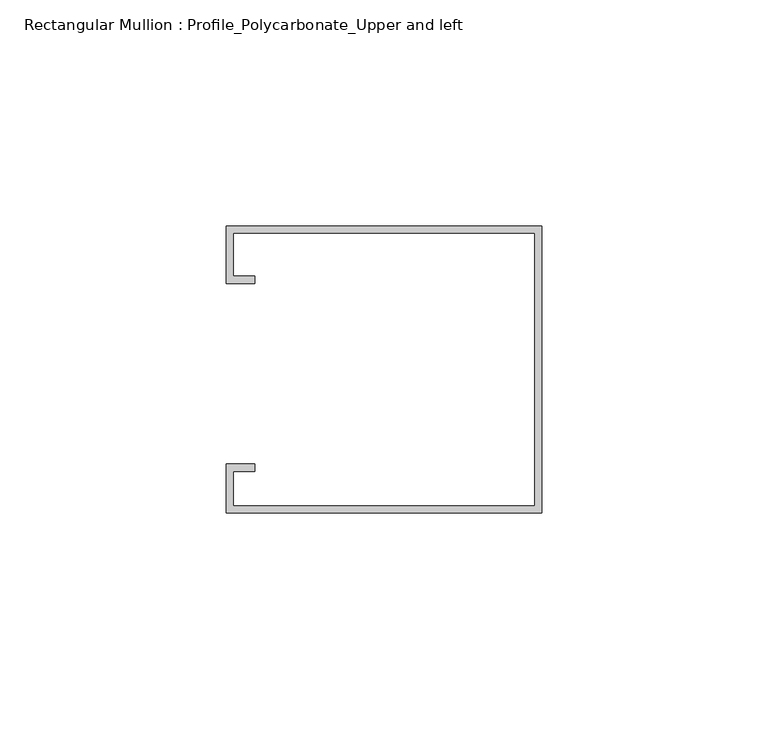
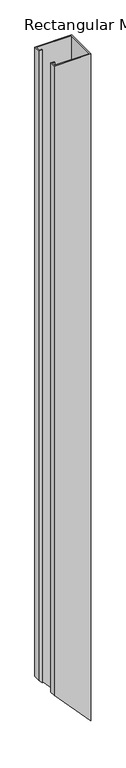
"""IFC4 building model written with IfcOpenShell, lengths in millimetres: member geometry, Rectangular Mullion : Profile_Polycarbonate_Upper and left."""

from ifc_helpers import new_model, si_unit, origin, place, context, project, spatial, faceted_brep, source, transform, mapped, element, save


def rectangular_mullion_profile_polycarbonate_upper_and_left_c3c58ff7(model_context):
    return source(origin(), model_context, "Body", "Brep", [
        faceted_brep([(0.0, 32.7, 0.0), (-69.85, 32.7, 0.0), (-69.85, 20.0, 0.0), (-63.5, 20.0, 0.0), (-63.5, 21.5875, 0.0), (-68.2625, 21.5875, 0.0), (-68.2625, 31.1125, 0.0), (-1.5875, 31.1125, 0.0), (-1.5875, -29.2125, 0.0), (-68.2625, -29.2125, 0.0), (-68.2625, -21.5875, 0.0), (-63.5, -21.5875, 0.0), (-63.5, -20.0, 0.0), (-69.85, -20.0, 0.0), (-69.85, -30.8, 0.0), (0.0, -30.8, 0.0), (0.0, 32.7, -1345.3170334), (-69.85, 32.7, -1269.404085), (-69.85, 20.0, -1269.404085), (-63.5, 20.0, -1276.3052621), (-63.5, 21.5875, -1276.3052621), (-68.2625, 21.5875, -1271.1293793), (-68.2625, 31.1125, -1271.1293793), (-1.5875, 31.1125, -1343.5917391), (-1.5875, -29.2125, -1343.5917391), (-68.2625, -29.2125, -1271.1293793), (-68.2625, -21.5875, -1271.1293793), (-63.5, -21.5875, -1276.3052621), (-63.5, -20.0, -1276.3052621), (-69.85, -20.0, -1269.404085), (-69.85, -30.8, -1269.404085), (0.0, -30.8, -1345.3170334)], [[[0, 1, 2, 3, 4, 5, 6, 7, 8, 9, 10, 11, 12, 13, 14, 15]], [[1, 0, 16, 17]], [[2, 1, 17, 18]], [[3, 2, 18, 19]], [[4, 3, 19, 20]], [[5, 4, 20, 21]], [[6, 5, 21, 22]], [[7, 6, 22, 23]], [[8, 7, 23, 24]], [[9, 8, 24, 25]], [[10, 9, 25, 26]], [[11, 10, 26, 27]], [[12, 11, 27, 28]], [[13, 12, 28, 29]], [[14, 13, 29, 30]], [[15, 14, 30, 31]], [[0, 15, 31, 16]], [[16, 31, 30, 29, 28, 27, 26, 25, 24, 23, 22, 21, 20, 19, 18, 17]]]),
    ])


if __name__ == "__main__":
    model = new_model("IFC4")
    model_context = context("Model", 3, world=origin())
    ifc_project = project(units=[si_unit("LENGTHUNIT", "METRE", prefix="MILLI")], contexts=[model_context])
    site = spatial("IfcSite", under=ifc_project)
    building = spatial("IfcBuilding", under=site)
    placement = place(None, origin())
    rectangular_mullion_profile_polycarbonate_upper_and_left_shape = rectangular_mullion_profile_polycarbonate_upper_and_left_c3c58ff7(model_context)
    element("IfcMember", 1, ObjectType="Rectangular Mullion : Profile_Polycarbonate_Upper and left", at=placement, inside=building, context=model_context, shape_type="MappedRepresentation", body=[
        mapped(rectangular_mullion_profile_polycarbonate_upper_and_left_shape, transform((0.0, 0.0, 0.0), x_axis=(1.0, 0.0, 0.0), y_axis=(0.0, 1.0, 0.0), z_axis=(0.0, 0.0, 1.0))),
    ])
    save(model, "model.ifc")

# Revit data of these elements
# Type "Rectangular Mullion : Profile_Polycarbonate_Upper and left"
#   built-in parameter 1007322 = 0.208333 (stored number, unit not read)
#   built-in parameter 1007321 = 0.00520833 (stored number, unit not read)
#   built-in parameter 1007320 = 0 (stored number, unit not read)
# Element 1 (IfcMember, "Rectangular Mullion : Profile_Polycarbonate_Upper and left")
#   Materials on its faces: "ALUMINUM PROFILE AT POLYCARBONATE PANEL"
# Materials
#   "ALUMINUM PROFILE AT POLYCARBONATE PANEL": class "Metal", colour RGB 244 244 244, transparency 0, Description = "Aluminum 6061", Cost = 0
